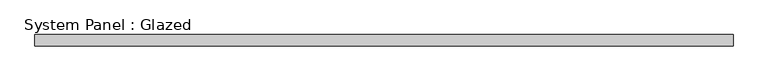
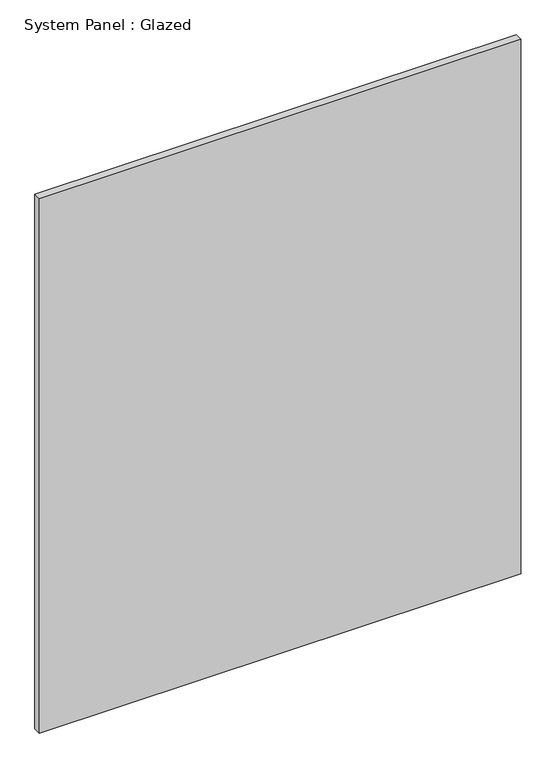
"""IFC4 building model written with IfcOpenShell, lengths in millimetres: plate geometry, System Panel : Glazed."""

from ifc_helpers import new_model, si_unit, origin, origin_with_axes, place, context, project, spatial, polyline, outline, extrude, source, transform, mapped, element, save


def system_panel_glazed_d066ac4e(model_context):
    return source(origin(), model_context, "Body", "SweptSolid", [
        extrude(outline(polyline([(782.8178526, 24.5), (-782.8178526, 24.5), (-782.8178526, 49.5), (782.8178526, 49.5), (782.8178526, 24.5)])), origin_with_axes(), (0.0, 0.0, 1.0), 1837.3779433),
    ])


if __name__ == "__main__":
    model = new_model("IFC4")
    model_context = context("Model", 3, world=origin())
    ifc_project = project(units=[si_unit("LENGTHUNIT", "METRE", prefix="MILLI")], contexts=[model_context])
    site = spatial("IfcSite", under=ifc_project)
    building = spatial("IfcBuilding", under=site)
    placement = place(None, origin())
    system_panel_glazed_shape = system_panel_glazed_d066ac4e(model_context)
    element("IfcPlate", 1, ObjectType="System Panel : Glazed", at=placement, inside=building, context=model_context, shape_type="MappedRepresentation", body=[
        mapped(system_panel_glazed_shape, transform((0.0, 0.0, 0.0), x_axis=(1.0, 0.0, 0.0), y_axis=(0.0, 1.0, 0.0), z_axis=(0.0, 0.0, 1.0))),
    ])
    save(model, "model.ifc")

# Revit data of these elements
# Element 1 (IfcPlate, "System Panel : Glazed")
#   Materials on its faces: "Glass"
# Materials
#   "Glass": class "Glass", colour RGB 218 227 224, transparency 0.85, Description = "Soda Lime Glass", Cost = 0
